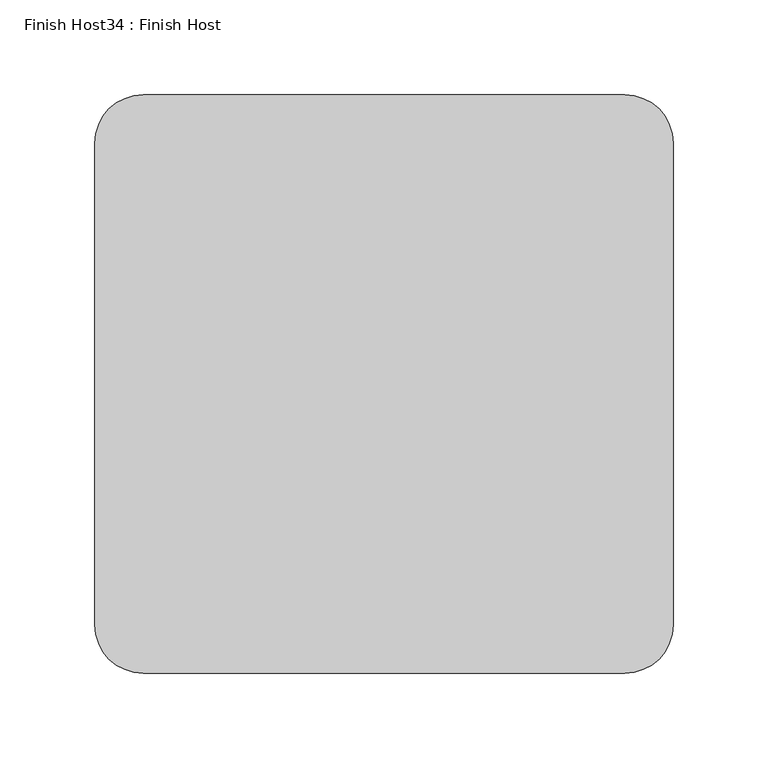
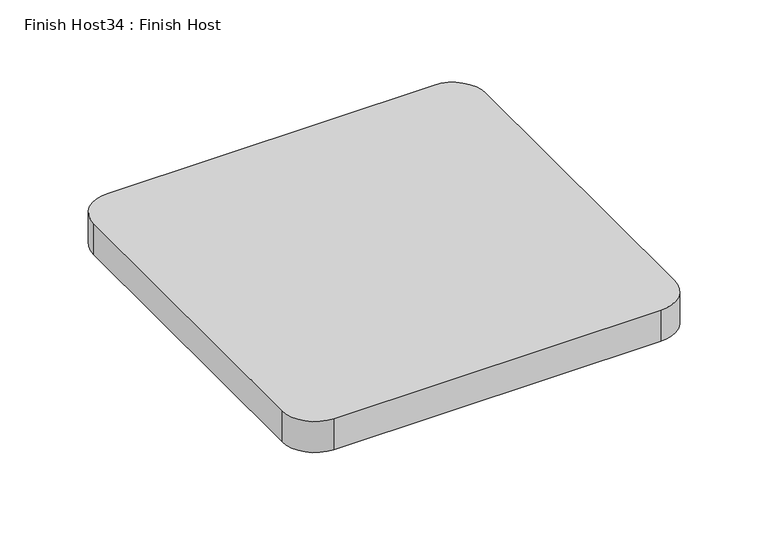
"""IFC4 building model written with IfcOpenShell, lengths in millimetres: proxy geometry, Finish Host34 : Finish Host."""

from ifc_helpers import new_model, si_unit, point, frame_2d, origin, origin_with_axes, place, context, project, spatial, polyline, circle_curve, trimmed, segment, composite_curve, outline, extrude, source, transform, mapped, element, save


def finish_host34_finish_host_3f4a88f0(model_context):
    return source(origin(), model_context, "Body", "SweptSolid", [
        extrude(outline(composite_curve([segment(polyline([(-14319.2939795, 14061.2419385), (-14319.2939795, 14315.2419385)]), True, "CONTINUOUS"), segment(trimmed(circle_curve(frame_2d((-14293.8939795, 14315.2419385)), 25.4), [point((-14319.2939795, 14315.2419385))], [point((-14293.8939795, 14340.6419385))], False, "CARTESIAN"), True, "CONTINUOUS"), segment(polyline([(-14293.8939795, 14340.6419385), (-14039.8939795, 14340.6419385)]), True, "CONTINUOUS"), segment(trimmed(circle_curve(frame_2d((-14039.8939795, 14315.2419385)), 25.4), [point((-14039.8939795, 14340.6419385))], [point((-14014.4939795, 14315.2419385))], False, "CARTESIAN"), True, "CONTINUOUS"), segment(polyline([(-14014.4939795, 14315.2419385), (-14014.4939795, 14061.2419385)]), True, "CONTINUOUS"), segment(trimmed(circle_curve(frame_2d((-14039.8939795, 14061.2419385)), 25.4), [point((-14014.4939795, 14061.2419385))], [point((-14039.8939795, 14035.8419385))], False, "CARTESIAN"), True, "CONTINUOUS"), segment(polyline([(-14039.8939795, 14035.8419385), (-14293.8939795, 14035.8419385)]), True, "CONTINUOUS"), segment(trimmed(circle_curve(frame_2d((-14293.8939795, 14061.2419385)), 25.4), [point((-14293.8939795, 14035.8419385))], [point((-14319.2939795, 14061.2419385))], False, "CARTESIAN"), True, "CONTINUOUS")], self_intersect=False)), origin_with_axes(), (0.0, 0.0, 1.0), 25.4),
    ])


if __name__ == "__main__":
    model = new_model("IFC4")
    model_context = context("Model", 3, world=origin())
    ifc_project = project(units=[si_unit("LENGTHUNIT", "METRE", prefix="MILLI")], contexts=[model_context])
    site = spatial("IfcSite", under=ifc_project)
    building = spatial("IfcBuilding", under=site)
    placement = place(None, origin())
    finish_host34_finish_host_shape = finish_host34_finish_host_3f4a88f0(model_context)
    element("IfcBuildingElementProxy", 1, Name="Finish Host34 : Finish Host", ObjectType="Finish Host34 : Finish Host", at=placement, inside=building, context=model_context, shape_type="MappedRepresentation", body=[
        mapped(finish_host34_finish_host_shape, transform((0.0, 0.0, 0.0), x_axis=(1.0, 0.0, 0.0), y_axis=(0.0, 1.0, 0.0), z_axis=(0.0, 0.0, 1.0))),
    ])
    save(model, "model.ifc")

# Revit data of these elements
# Type "Finish Host34 : Finish Host"
#   Panel Material = none
# Element 1 (IfcBuildingElementProxy, "Finish Host34 : Finish Host")
#   Materials on its faces: "Thread - Teknion - Navy"
# Materials
#   "Thread - Teknion - Navy": class "Fabric", colour RGB 28 32 67, transparency 0, Model = "F206", Manufacturer = "Teknion Studio", URL = "http://www.teknion.com/", Description = "Fantasme Full Wool", Cost = 0
